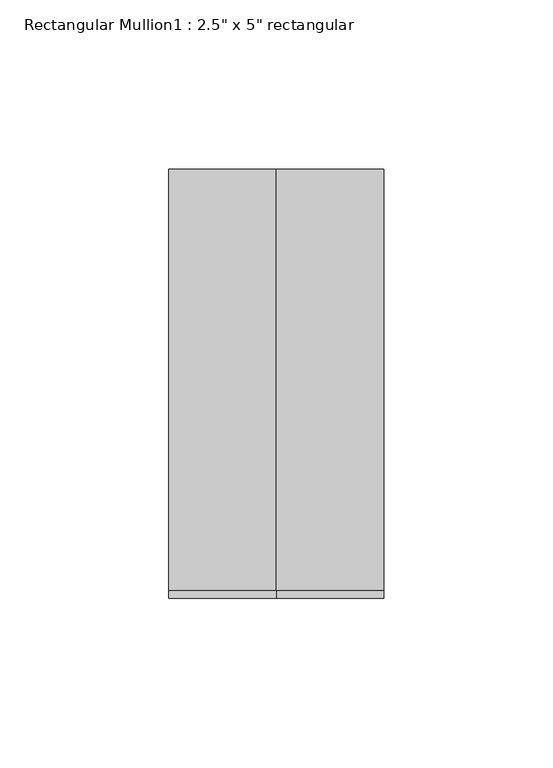
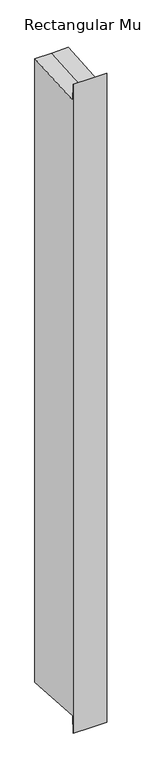
"""IFC4 building model written with IfcOpenShell, lengths in millimetres: member geometry."""

from ifc_helpers import new_model, si_unit, origin, place, context, project, spatial, faceted_brep, source, transform, mapped, element, save


def member_9c235780(model_context):
    return source(origin(), model_context, "Body", "Brep", [
        faceted_brep([(-31.75, 63.5, 4.2249441), (0.0, 63.5, 4.2249441), (31.75, 63.5, 4.2249441), (31.75, 63.5, -1253.4859011), (0.0, 63.5, -1253.4859011), (-31.75, 63.5, -1253.4859011), (-31.75, -63.5, 29.6036678), (-31.75, -61.2111885, -4.2153013), (-31.75, -61.2111885, -1245.0456557), (-31.75, -63.5, -1278.8646248), (31.75, -63.5, 29.6036678), (0.0, -63.5, 29.6036678), (0.0, -63.5, -1278.8646248), (31.75, -63.5, -1278.8646248), (31.75, -61.2111885, -4.2153013), (31.75, -61.2111885, -1245.0456557), (0.0, -61.2111885, -4.2153013), (0.0, -61.2111885, -1245.0456557)], [[[0, 1, 2, 3, 4, 5]], [[6, 7, 0, 5, 8, 9]], [[10, 11, 6, 9, 12, 13]], [[2, 14, 10, 13, 15, 3]], [[2, 1, 16, 14]], [[1, 0, 7, 16]], [[7, 6, 11, 16]], [[11, 10, 14, 16]], [[3, 15, 17, 4]], [[15, 13, 12, 17]], [[12, 9, 8, 17]], [[8, 5, 4, 17]]]),
    ])


if __name__ == "__main__":
    model = new_model("IFC4")
    model_context = context("Model", 3, world=origin())
    ifc_project = project(units=[si_unit("LENGTHUNIT", "METRE", prefix="MILLI")], contexts=[model_context])
    site = spatial("IfcSite", under=ifc_project)
    building = spatial("IfcBuilding", under=site)
    placement = place(None, origin())
    member_shape = member_9c235780(model_context)
    element("IfcMember", 1, ObjectType="Rectangular Mullion1 : 2.5\" x 5\" rectangular", at=placement, inside=building, context=model_context, shape_type="MappedRepresentation", body=[
        mapped(member_shape, transform((0.0, 0.0, 0.0), x_axis=(1.0, 0.0, 0.0), y_axis=(0.0, 1.0, 0.0), z_axis=(0.0, 0.0, 1.0))),
    ])
    save(model, "model.ifc")

# Revit data of these elements
# Type "Rectangular Mullion1 : 2.5\" x 5\" rectangular"
#   built-in parameter 1007304 = 0.416667 (stored number, unit not read)
#   built-in parameter 1007301 = 0.104167 (stored number, unit not read)
#   built-in parameter 1007300 = 0.104167 (stored number, unit not read)
# Element 1 (IfcMember, "Rectangular Mullion1 : 2.5\" x 5\" rectangular")
#   Materials on its faces: "support-frame"
# Materials
#   "support-frame": class "Unassigned", colour RGB 233 233 233, transparency 0, Cost = 0
